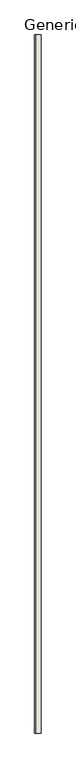
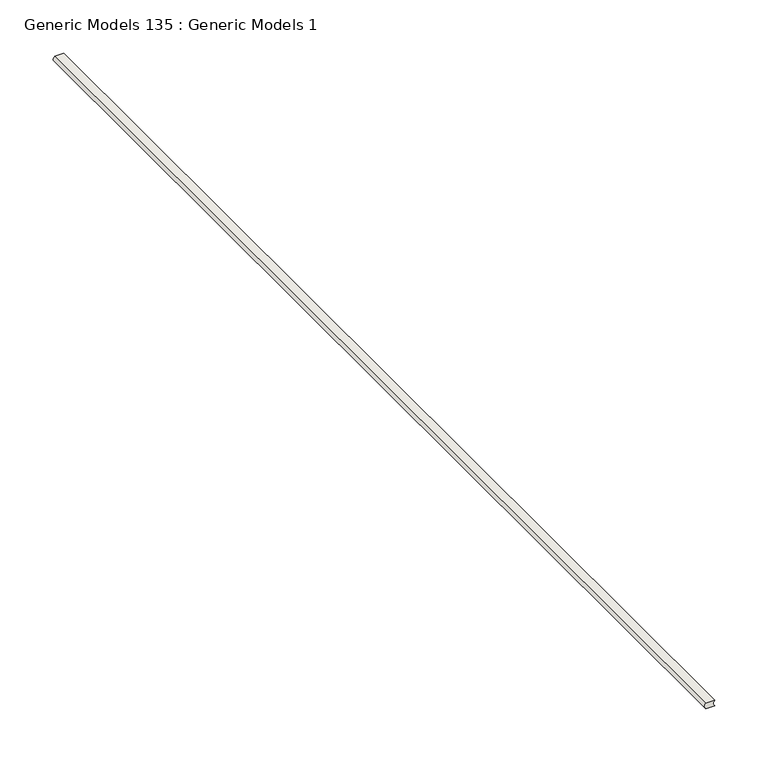
"""IFC4 building model written with IfcOpenShell, lengths in millimetres: wall geometry, Generic Models 135 : Generic Models 1."""

from ifc_helpers import new_model, si_unit, point, frame, frame_2d, origin, place, context, project, spatial, polyline, circle_curve, trimmed, segment, composite_curve, outline, extrude, source, transform, mapped, element, save


def generic_models_135_generic_models_1_c2654668(model_context):
    return source(origin(), model_context, "Body", "SweptSolid", [
        extrude(outline(composite_curve([segment(trimmed(circle_curve(frame_2d((3.175, 51017.2271135)), 4.3100275), [point((0.0, 51014.312373))], [point((6.35, 51014.312373))], True, "CARTESIAN"), True, "CONTINUOUS"), segment(polyline([(6.35, 51014.312373), (6.35, 51004.787373)]), True, "CONTINUOUS"), segment(trimmed(circle_curve(frame_2d((3.175, 51007.7021135)), 4.3100275), [point((6.35, 51004.787373))], [point((0.0, 51004.787373))], False, "CARTESIAN"), True, "CONTINUOUS"), segment(polyline([(0.0, 51004.787373), (0.0, 51014.312373)]), True, "CONTINUOUS")], self_intersect=False)), frame((0.0, 0.0, 0.0), z_axis=(0.0, 1.0, 0.0), x_axis=(0.0, 0.0, 1.0)), (0.0, 0.0, 1.0), 1219.2),
    ])


if __name__ == "__main__":
    model = new_model("IFC4")
    model_context = context("Model", 3, world=origin())
    ifc_project = project(units=[si_unit("LENGTHUNIT", "METRE", prefix="MILLI")], contexts=[model_context])
    site = spatial("IfcSite", under=ifc_project)
    building = spatial("IfcBuilding", under=site)
    placement = place(None, origin())
    generic_models_135_generic_models_1_shape = generic_models_135_generic_models_1_c2654668(model_context)
    element("IfcWall", 1, ObjectType="Generic Models 135 : Generic Models 1", at=placement, inside=building, context=model_context, shape_type="MappedRepresentation", body=[
        mapped(generic_models_135_generic_models_1_shape, transform((0.0, 0.0, 0.0), x_axis=(1.0, 0.0, 0.0), y_axis=(0.0, 1.0, 0.0), z_axis=(0.0, 0.0, 1.0))),
    ])
    save(model, "model.ifc")

# Revit data of these elements
# Element 1 (IfcWall, "Generic Models 135 : Generic Models 1")
#   Materials on its faces: "SEALANT (W/ BACKER ROD IF NECESSARY)"
# Materials
#   "SEALANT (W/ BACKER ROD IF NECESSARY)": class "Unassigned", colour RGB 120 120 120, transparency 0, Cost = 0
